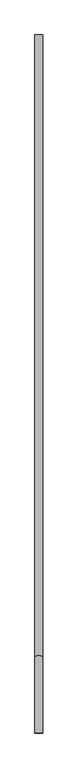
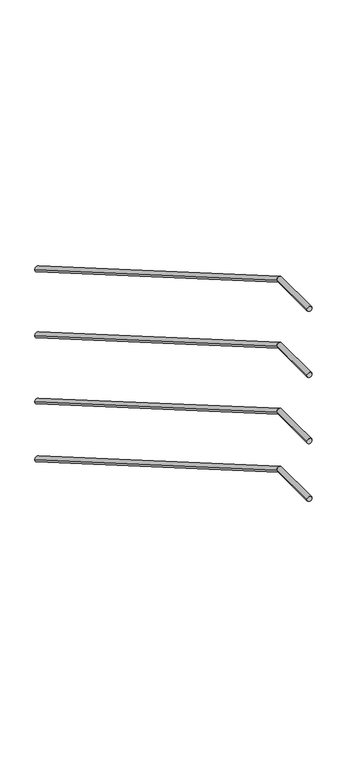
"""IFC4 building model written with IfcOpenShell, lengths in millimetres: railing geometry."""

from ifc_helpers import new_model, si_unit, frame, origin, place, context, project, spatial, circle_curve, ellipse_curve, source, transform, mapped, element, save
from ifc_brep_helpers import plane_surface, cylinder_surface, advanced_brep


def railing_cad50a57(model_context):
    return source(origin(), model_context, "Body", "AdvancedBrep", [
        advanced_brep(
        [(-1709.6, 15799.5208589, 2729.6773196), (-1739.6, 15799.5208589, 2729.6773196), (-1709.6, 13395.4833005, 4124.9618634), (-1739.6, 13395.4833005, 4124.9618634), (-1709.6, 13099.5208589, 4124.9618634), (-1739.6, 13099.5208589, 4124.9618634)],
        [
            (0, 1, ellipse_curve(frame((-1724.6, 15799.5208589, 2729.6773196), z_axis=(0.0, 1.0, 0.0), x_axis=(0.0, 0.0, -1.0)), 17.3433672, 15.0)),
            (1, 0, ellipse_curve(frame((-1724.6, 15799.5208589, 2729.6773196), z_axis=(0.0, 1.0, 0.0), x_axis=(0.0, 0.0, -1.0)), 17.3433672, 15.0)),
            (0, 2),
            (2, 3, ellipse_curve(frame((-1724.6, 13395.4833005, 4124.9618634), z_axis=(0.0, 0.9656303515230847, -0.25991926480621563), x_axis=(0.0, -0.25991926480621524, -0.9656303515230849)), 15.5338945, 15.0)),
            (3, 1),
            (3, 2, ellipse_curve(frame((-1724.6, 13395.4833005, 4124.9618634), z_axis=(0.0, 0.9656303515230847, -0.25991926480621563), x_axis=(0.0, -0.25991926480621524, -0.9656303515230849)), 15.5338945, 15.0)),
            (4, 5, circle_curve(frame((-1724.6, 13099.5208589, 4124.9618634), z_axis=(0.0, -1.0, 0.0), x_axis=(-1.0, 0.0, 0.0)), 15.0)),
            (5, 4, circle_curve(frame((-1724.6, 13099.5208589, 4124.9618634), z_axis=(0.0, -1.0, 0.0), x_axis=(-1.0, 0.0, 0.0)), 15.0)),
            (2, 4),
            (5, 3),
        ],
        [
            plane_surface(frame((-1724.6, 15799.5208589, 2747.0206869), z_axis=(0.0, 1.0, 0.0), x_axis=(0.0, 0.0, -1.0))),
            cylinder_surface(frame((-1724.6, 15791.991281, 2734.0474276), z_axis=(0.0, 0.8648839515651927, -0.5019718620848955), x_axis=(-1.0, 0.0, 0.0)), 15.0),
            plane_surface(frame((-1724.6, 13099.5208589, 4139.9618634), z_axis=(0.0, -1.0, 0.0), x_axis=(0.0, 0.0, -1.0))),
            cylinder_surface(frame((-1724.6, 13399.5208589, 4124.9618634), z_axis=(0.0, 1.0, 0.0), x_axis=(-1.0, 0.0, 0.0)), 15.0),
        ],
        [
            (0, [[1, 2]]),
            (1, [[-1, 3, 4, 5]]),
            (1, [[-2, -5, 6, -3]]),
            (2, [[7, 8]]),
            (3, [[-4, 9, -8, 10]]),
            (3, [[-6, -10, -7, -9]]),
        ],
    ),
        advanced_brep(
        [(-1709.6, 15799.5208589, 1929.6773196), (-1739.6, 15799.5208589, 1929.6773196), (-1709.6, 13395.4833005, 3324.9618634), (-1739.6, 13395.4833005, 3324.9618634), (-1709.6, 13099.5208589, 3324.9618634), (-1739.6, 13099.5208589, 3324.9618634)],
        [
            (0, 1, ellipse_curve(frame((-1724.6, 15799.5208589, 1929.6773196), z_axis=(0.0, 1.0, 0.0), x_axis=(0.0, 0.0, -1.0)), 17.3433672, 15.0)),
            (1, 0, ellipse_curve(frame((-1724.6, 15799.5208589, 1929.6773196), z_axis=(0.0, 1.0, 0.0), x_axis=(0.0, 0.0, -1.0)), 17.3433672, 15.0)),
            (0, 2),
            (2, 3, ellipse_curve(frame((-1724.6, 13395.4833005, 3324.9618634), z_axis=(0.0, 0.9656303515230847, -0.25991926480621563), x_axis=(0.0, -0.25991926480621524, -0.9656303515230849)), 15.5338945, 15.0)),
            (3, 1),
            (3, 2, ellipse_curve(frame((-1724.6, 13395.4833005, 3324.9618634), z_axis=(0.0, 0.9656303515230847, -0.25991926480621563), x_axis=(0.0, -0.25991926480621524, -0.9656303515230849)), 15.5338945, 15.0)),
            (4, 5, circle_curve(frame((-1724.6, 13099.5208589, 3324.9618634), z_axis=(0.0, -1.0, 0.0), x_axis=(-1.0, 0.0, 0.0)), 15.0)),
            (5, 4, circle_curve(frame((-1724.6, 13099.5208589, 3324.9618634), z_axis=(0.0, -1.0, 0.0), x_axis=(-1.0, 0.0, 0.0)), 15.0)),
            (2, 4),
            (5, 3),
        ],
        [
            plane_surface(frame((-1724.6, 15799.5208589, 1947.0206869), z_axis=(0.0, 1.0, 0.0), x_axis=(0.0, 0.0, -1.0))),
            cylinder_surface(frame((-1724.6, 15791.991281, 1934.0474276), z_axis=(0.0, 0.8648839515651927, -0.5019718620848955), x_axis=(-1.0, 0.0, 0.0)), 15.0),
            plane_surface(frame((-1724.6, 13099.5208589, 3339.9618634), z_axis=(0.0, -1.0, 0.0), x_axis=(0.0, 0.0, -1.0))),
            cylinder_surface(frame((-1724.6, 13399.5208589, 3324.9618634), z_axis=(0.0, 1.0, 0.0), x_axis=(-1.0, 0.0, 0.0)), 15.0),
        ],
        [
            (0, [[1, 2]]),
            (1, [[-1, 3, 4, 5]]),
            (1, [[-2, -5, 6, -3]]),
            (2, [[7, 8]]),
            (3, [[-4, 9, -8, 10]]),
            (3, [[-6, -10, -7, -9]]),
        ],
    ),
        advanced_brep(
        [(-1709.6, 15799.5208589, 2329.6773196), (-1739.6, 15799.5208589, 2329.6773196), (-1709.6, 13395.4833005, 3724.9618634), (-1739.6, 13395.4833005, 3724.9618634), (-1709.6, 13099.5208589, 3724.9618634), (-1739.6, 13099.5208589, 3724.9618634)],
        [
            (0, 1, ellipse_curve(frame((-1724.6, 15799.5208589, 2329.6773196), z_axis=(0.0, 1.0, 0.0), x_axis=(0.0, 0.0, -1.0)), 17.3433672, 15.0)),
            (1, 0, ellipse_curve(frame((-1724.6, 15799.5208589, 2329.6773196), z_axis=(0.0, 1.0, 0.0), x_axis=(0.0, 0.0, -1.0)), 17.3433672, 15.0)),
            (0, 2),
            (2, 3, ellipse_curve(frame((-1724.6, 13395.4833005, 3724.9618634), z_axis=(0.0, 0.9656303515230847, -0.25991926480621563), x_axis=(0.0, -0.25991926480621524, -0.9656303515230849)), 15.5338945, 15.0)),
            (3, 1),
            (3, 2, ellipse_curve(frame((-1724.6, 13395.4833005, 3724.9618634), z_axis=(0.0, 0.9656303515230847, -0.25991926480621563), x_axis=(0.0, -0.25991926480621524, -0.9656303515230849)), 15.5338945, 15.0)),
            (4, 5, circle_curve(frame((-1724.6, 13099.5208589, 3724.9618634), z_axis=(0.0, -1.0, 0.0), x_axis=(-1.0, 0.0, 0.0)), 15.0)),
            (5, 4, circle_curve(frame((-1724.6, 13099.5208589, 3724.9618634), z_axis=(0.0, -1.0, 0.0), x_axis=(-1.0, 0.0, 0.0)), 15.0)),
            (2, 4),
            (5, 3),
        ],
        [
            plane_surface(frame((-1724.6, 15799.5208589, 2347.0206869), z_axis=(0.0, 1.0, 0.0), x_axis=(0.0, 0.0, -1.0))),
            cylinder_surface(frame((-1724.6, 15791.991281, 2334.0474276), z_axis=(0.0, 0.8648839515651927, -0.5019718620848955), x_axis=(-1.0, 0.0, 0.0)), 15.0),
            plane_surface(frame((-1724.6, 13099.5208589, 3739.9618634), z_axis=(0.0, -1.0, 0.0), x_axis=(0.0, 0.0, -1.0))),
            cylinder_surface(frame((-1724.6, 13399.5208589, 3724.9618634), z_axis=(0.0, 1.0, 0.0), x_axis=(-1.0, 0.0, 0.0)), 15.0),
        ],
        [
            (0, [[1, 2]]),
            (1, [[-1, 3, 4, 5]]),
            (1, [[-2, -5, 6, -3]]),
            (2, [[7, 8]]),
            (3, [[-4, 9, -8, 10]]),
            (3, [[-6, -10, -7, -9]]),
        ],
    ),
        advanced_brep(
        [(-1709.6, 15799.5208589, 1579.6773196), (-1739.6, 15799.5208589, 1579.6773196), (-1709.6, 13395.4833005, 2974.9618634), (-1739.6, 13395.4833005, 2974.9618634), (-1709.6, 13099.5208589, 2974.9618634), (-1739.6, 13099.5208589, 2974.9618634)],
        [
            (0, 1, ellipse_curve(frame((-1724.6, 15799.5208589, 1579.6773196), z_axis=(0.0, 1.0, 0.0), x_axis=(0.0, 0.0, -1.0)), 17.3433672, 15.0)),
            (1, 0, ellipse_curve(frame((-1724.6, 15799.5208589, 1579.6773196), z_axis=(0.0, 1.0, 0.0), x_axis=(0.0, 0.0, -1.0)), 17.3433672, 15.0)),
            (0, 2),
            (2, 3, ellipse_curve(frame((-1724.6, 13395.4833005, 2974.9618634), z_axis=(0.0, 0.9656303515230847, -0.25991926480621563), x_axis=(0.0, -0.25991926480621524, -0.9656303515230849)), 15.5338945, 15.0)),
            (3, 1),
            (3, 2, ellipse_curve(frame((-1724.6, 13395.4833005, 2974.9618634), z_axis=(0.0, 0.9656303515230847, -0.25991926480621563), x_axis=(0.0, -0.25991926480621524, -0.9656303515230849)), 15.5338945, 15.0)),
            (4, 5, circle_curve(frame((-1724.6, 13099.5208589, 2974.9618634), z_axis=(0.0, -1.0, 0.0), x_axis=(-1.0, 0.0, 0.0)), 15.0)),
            (5, 4, circle_curve(frame((-1724.6, 13099.5208589, 2974.9618634), z_axis=(0.0, -1.0, 0.0), x_axis=(-1.0, 0.0, 0.0)), 15.0)),
            (2, 4),
            (5, 3),
        ],
        [
            plane_surface(frame((-1724.6, 15799.5208589, 1597.0206869), z_axis=(0.0, 1.0, 0.0), x_axis=(0.0, 0.0, -1.0))),
            cylinder_surface(frame((-1724.6, 15791.991281, 1584.0474276), z_axis=(0.0, 0.8648839515651927, -0.5019718620848955), x_axis=(-1.0, 0.0, 0.0)), 15.0),
            plane_surface(frame((-1724.6, 13099.5208589, 2989.9618634), z_axis=(0.0, -1.0, 0.0), x_axis=(0.0, 0.0, -1.0))),
            cylinder_surface(frame((-1724.6, 13399.5208589, 2974.9618634), z_axis=(0.0, 1.0, 0.0), x_axis=(-1.0, 0.0, 0.0)), 15.0),
        ],
        [
            (0, [[1, 2]]),
            (1, [[-1, 3, 4, 5]]),
            (1, [[-2, -5, 6, -3]]),
            (2, [[7, 8]]),
            (3, [[-4, 9, -8, 10]]),
            (3, [[-6, -10, -7, -9]]),
        ],
    ),
    ])


if __name__ == "__main__":
    model = new_model("IFC4")
    model_context = context("Model", 3, world=origin())
    ifc_project = project(units=[si_unit("LENGTHUNIT", "METRE", prefix="MILLI")], contexts=[model_context])
    site = spatial("IfcSite", under=ifc_project)
    building = spatial("IfcBuilding", under=site)
    placement = place(None, origin())
    railing_shape = railing_cad50a57(model_context)
    element("IfcRailing", 1, at=placement, inside=building, context=model_context, shape_type="MappedRepresentation", body=[
        mapped(railing_shape, transform((0.0, 0.0, 0.0), x_axis=(1.0, 0.0, 0.0), y_axis=(0.0, 1.0, 0.0), z_axis=(0.0, 0.0, 1.0))),
    ])
    save(model, "model.ifc")
